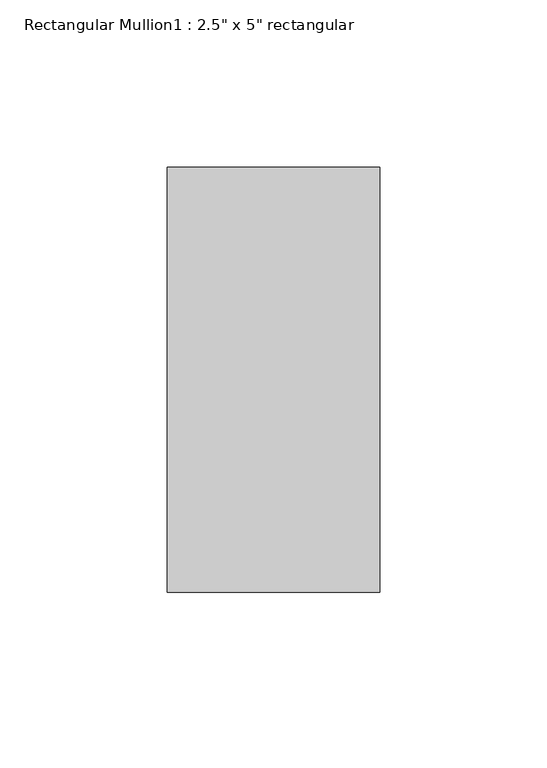
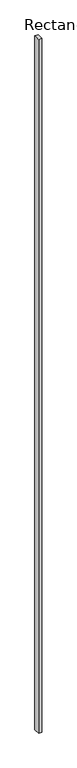
"""IFC4 building model written with IfcOpenShell, lengths in millimetres: member geometry."""

import ifcopenshell
import ifcopenshell.guid

model = None  # the IFC model being written
_history = None  # IfcOwnerHistory: only IFC2X3 demands one
_inside = {}  # id of a spatial element -> (the spatial element, [elements in it])
_under = {}  # id of a project, library or spatial element -> (it, [spatial elements below it])
_declared = {}  # id of a project -> (the project, [libraries it declares])
_typed = {}  # id of a type object -> (the type object, [elements of that type])
_made_of = {}  # id of a material, layer set ... -> (it, [elements and type objects made of it])


def new_model(schema):
    """Start an empty IFC model of exactly this schema.

    Asked for "IFC4X3", IfcOpenShell would pick the latest addendum, in which some entities
    have other attributes; the version numbers below select the first issue.
    IFC2X3 requires an IfcOwnerHistory on every rooted entity: one is made here for all.
    """
    global model, _history
    if schema == "IFC4X3":
        model = ifcopenshell.file(schema_version=(4, 3, 0, 0))
    else:
        model = ifcopenshell.file(schema=schema)
    _inside.clear()
    _under.clear()
    _declared.clear()
    _typed.clear()
    _made_of.clear()
    _history = None
    if model.schema == "IFC2X3":
        org = make("IfcOrganization", Name="unknown")
        user = make(
            "IfcPersonAndOrganization",
            ThePerson=make("IfcPerson", FamilyName="unknown"),
            TheOrganization=org,
        )
        app = make(
            "IfcApplication",
            ApplicationDeveloper=org,
            Version="unknown",
            ApplicationFullName="unknown",
            ApplicationIdentifier="unknown",
        )
        _history = make(
            "IfcOwnerHistory",
            OwningUser=user,
            OwningApplication=app,
            ChangeAction="ADDED",
            CreationDate=0,
        )
    return model


def make(cls, **values):
    """One entity of the class cls with the attributes given. An attribute that is None is left unset."""
    return model.create_entity(
        cls, **{name: value for name, value in values.items() if value is not None}
    )


def rooted(cls, **values):
    """An entity with a GlobalId (a new one), such as an element, a storey or a relation."""
    return make(cls, GlobalId=ifcopenshell.guid.new(), OwnerHistory=_history, **values)


def si_unit(unit_type, name, prefix=None):
    """IfcSIUnit, for example si_unit("LENGTHUNIT", "METRE", prefix="MILLI")."""
    return make("IfcSIUnit", UnitType=unit_type, Prefix=prefix, Name=name)


def assignment(units):
    """IfcUnitAssignment: the units of a project."""
    return None if units is None else make("IfcUnitAssignment", Units=units)


def point(xyz):
    """IfcCartesianPoint."""
    return None if xyz is None else make("IfcCartesianPoint", Coordinates=xyz)


def direction(xyz):
    """IfcDirection."""
    return None if xyz is None else make("IfcDirection", DirectionRatios=xyz)


def frame(location, z_axis=None, x_axis=None):
    """IfcAxis2Placement3D, a coordinate frame: its origin and axes. An axis left out is left unset."""
    return make(
        "IfcAxis2Placement3D",
        Location=point(location),
        Axis=direction(z_axis),
        RefDirection=direction(x_axis),
    )


def origin():
    """The frame at (0, 0, 0) with its axes left unset."""
    return frame((0.0, 0.0, 0.0))


def place(relative_to, where):
    """IfcLocalPlacement: puts the frame where relative to a parent placement (None: the world)."""
    return make(
        "IfcLocalPlacement", PlacementRelTo=relative_to, RelativePlacement=where
    )


def context(
    kind, dimensions, precision=None, world=None, true_north=None, identifier=None
):
    """IfcGeometricRepresentationContext, for example the 3D "Model" context."""
    return make(
        "IfcGeometricRepresentationContext",
        ContextIdentifier=identifier,
        ContextType=kind,
        CoordinateSpaceDimension=dimensions,
        Precision=precision,
        WorldCoordinateSystem=world,
        TrueNorth=true_north,
    )


def project(units=None, contexts=None):
    """IfcProject with its units and contexts."""
    return rooted(
        "IfcProject",
        Name="project",
        RepresentationContexts=contexts,
        UnitsInContext=assignment(units),
    )


def spatial(cls, under=None, at=None, **own):
    """A site, building, storey or space (cls), placed at a placement, below another one or the project."""
    s = rooted(cls, ObjectPlacement=at, **own)
    if under is not None:
        _under.setdefault(under.id(), (under, []))[1].append(s)
    return s


def polyline(points):
    """IfcPolyline through the points."""
    return make("IfcPolyline", Points=[point(p) for p in points])


def outline(outer, holes=None, kind="AREA"):
    """IfcArbitraryClosedProfileDef: a profile drawn as a closed curve; with holes, ...WithVoids."""
    if holes is None:
        return make("IfcArbitraryClosedProfileDef", ProfileType=kind, OuterCurve=outer)
    return make(
        "IfcArbitraryProfileDefWithVoids",
        ProfileType=kind,
        OuterCurve=outer,
        InnerCurves=holes,
    )


def extrude(swept, where, along, depth):
    """IfcExtrudedAreaSolid: the profile swept, set in the frame where, extruded along a direction by depth."""
    return make(
        "IfcExtrudedAreaSolid",
        SweptArea=swept,
        Position=where,
        ExtrudedDirection=direction(along),
        Depth=depth,
    )


def shape(context_of_items, identifier, shape_type, items):
    """IfcShapeRepresentation: the items that make up one representation, for example the "Body"."""
    return make(
        "IfcShapeRepresentation",
        ContextOfItems=context_of_items,
        RepresentationIdentifier=identifier,
        RepresentationType=shape_type,
        Items=items,
    )


def source(mapping_origin, context_of_items, identifier, shape_type, items):
    """IfcRepresentationMap: a shape defined once, which mapped items show again and again."""
    return make(
        "IfcRepresentationMap",
        MappingOrigin=mapping_origin,
        MappedRepresentation=shape(context_of_items, identifier, shape_type, items),
    )


def transform(
    local_origin,
    x_axis=None,
    y_axis=None,
    z_axis=None,
    scale=None,
    scale2=None,
    scale3=None,
    uniform=True,
):
    """IfcCartesianTransformationOperator3D, or its non-uniform kind. x_axis, y_axis, z_axis: its Axis1, 2, 3."""
    if uniform:
        return make(
            "IfcCartesianTransformationOperator3D",
            Axis1=direction(x_axis),
            Axis2=direction(y_axis),
            LocalOrigin=point(local_origin),
            Scale=scale,
            Axis3=direction(z_axis),
        )
    return make(
        "IfcCartesianTransformationOperator3DnonUniform",
        Axis1=direction(x_axis),
        Axis2=direction(y_axis),
        LocalOrigin=point(local_origin),
        Scale=scale,
        Axis3=direction(z_axis),
        Scale2=scale2,
        Scale3=scale3,
    )


def mapped(mapping_source, mapping_target):
    """IfcMappedItem: shows the shape of a source again, moved by a transform."""
    return make(
        "IfcMappedItem", MappingSource=mapping_source, MappingTarget=mapping_target
    )


def made_of(thing, what):
    """Note that an element or type object is made of a material, layer set ...; save() writes the relation."""
    if what is not None:
        _made_of.setdefault(what.id(), (what, []))[1].append(thing)
    return thing


def element(
    cls,
    number,
    at=None,
    inside=None,
    cuts=None,
    type_object=None,
    material=None,
    context=None,
    identifier="Body",
    shape_type=None,
    held_by="IfcProductDefinitionShape",
    body=None,
    shapes=None,
    **own,
):
    """One element of the class cls, such as IfcWall. Its Tag is "e" and its number.

    at: its placement. inside: the storey or other place that contains it. cuts: it is an
    opening in that element (IfcRelVoidsElement). A single representation is given by context,
    identifier, shape_type and body (its items); several are given by shapes. held_by: the class
    of the entity that holds the representations. save() writes the other relations.
    """
    e = rooted(cls, Tag="e%d" % number, ObjectPlacement=at, **own)
    if body is not None:
        shapes = [shape(context, identifier, shape_type, body)]
    if shapes is not None:
        e.Representation = make(held_by, Representations=shapes)
    if inside is not None:
        _inside.setdefault(inside.id(), (inside, []))[1].append(e)
    if cuts is not None:
        rooted(
            "IfcRelVoidsElement", RelatingBuildingElement=cuts, RelatedOpeningElement=e
        )
    if type_object is not None:
        _typed.setdefault(type_object.id(), (type_object, []))[1].append(e)
    return made_of(e, material)


def aggregate(whole, parts):
    """IfcRelAggregates: a whole, such as a stair, and the parts it consists of."""
    return rooted("IfcRelAggregates", RelatingObject=whole, RelatedObjects=parts)


def save(model, path):
    """Write the relations noted so far, then the file.

    IfcRelAggregates (storeys below a building ...), IfcRelContainedInSpatialStructure (elements
    in a storey), IfcRelDefinesByType, IfcRelAssociatesMaterial and IfcRelDeclares: one each for
    every whole, place, type object, material and project.
    """
    for whole, parts in _under.values():
        aggregate(whole, parts)
    for where, things in _inside.values():
        rooted(
            "IfcRelContainedInSpatialStructure",
            RelatedElements=things,
            RelatingStructure=where,
        )
    for kind, things in _typed.values():
        rooted("IfcRelDefinesByType", RelatedObjects=things, RelatingType=kind)
    for what, things in _made_of.values():
        rooted("IfcRelAssociatesMaterial", RelatedObjects=things, RelatingMaterial=what)
    for by, libraries in _declared.values():
        rooted("IfcRelDeclares", RelatingContext=by, RelatedDefinitions=libraries)
    model.write(path)


def member_bd9c79d2(model_context):
    return source(origin(), model_context, "Body", "SweptSolid", [
        extrude(outline(polyline([(0.0, 63.5), (0.0, -63.5), (-63.5, -63.5), (-63.5, 63.5), (0.0, 63.5)])), frame((0.0, 0.0, -14960.6), z_axis=(0.0, 0.0, 1.0), x_axis=(1.0, 0.0, 0.0)), (0.0, 0.0, 1.0), 14960.6),
    ])


if __name__ == "__main__":
    model = new_model("IFC4")
    model_context = context("Model", 3, world=origin())
    ifc_project = project(units=[si_unit("LENGTHUNIT", "METRE", prefix="MILLI")], contexts=[model_context])
    site = spatial("IfcSite", under=ifc_project)
    building = spatial("IfcBuilding", under=site)
    placement = place(None, origin())
    member_shape = member_bd9c79d2(model_context)
    element("IfcMember", 1, ObjectType="Rectangular Mullion1 : 2.5\" x 5\" rectangular", at=placement, inside=building, context=model_context, shape_type="MappedRepresentation", body=[
        mapped(member_shape, transform((0.0, 0.0, 0.0), x_axis=(1.0, 0.0, 0.0), y_axis=(0.0, 1.0, 0.0), z_axis=(0.0, 0.0, 1.0))),
    ])
    save(model, "model.ifc")

# Revit data of these elements
# Type "Rectangular Mullion1 : 2.5\" x 5\" rectangular"
#   built-in parameter 1007304 = 0.416667 (stored number, unit not read)
#   built-in parameter 1007301 = 0.104167 (stored number, unit not read)
#   built-in parameter 1007300 = 0.104167 (stored number, unit not read)
# Element 1 (IfcMember, "Rectangular Mullion1 : 2.5\" x 5\" rectangular")
#   Materials on its faces: "support-frame"
# Materials
#   "support-frame": class "Unassigned", colour RGB 233 233 233, transparency 0, Cost = 0
